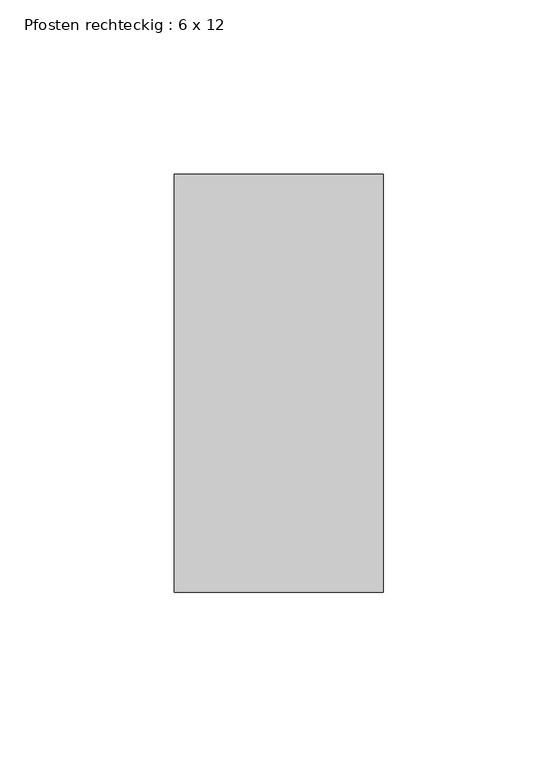
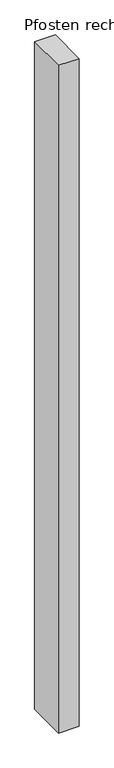
"""IFC4 building model written with IfcOpenShell, lengths in millimetres: member geometry, Pfosten rechteckig : 6 x 12."""

from ifc_helpers import new_model, si_unit, frame, origin, place, context, project, spatial, polyline, outline, extrude, source, transform, mapped, element, save


def pfosten_rechteckig_6_x_12_0a3b7900(model_context):
    return source(origin(), model_context, "Body", "SweptSolid", [
        extrude(outline(polyline([(0.0, 60.0), (0.0, -60.0), (-60.0, -60.0), (-60.0, 60.0), (0.0, 60.0)])), frame((0.0, 0.0, -2050.0000003), z_axis=(0.0, 0.0, 1.0), x_axis=(1.0, 0.0, 0.0)), (0.0, 0.0, 1.0), 2050.0000003),
    ])


if __name__ == "__main__":
    model = new_model("IFC4")
    model_context = context("Model", 3, world=origin())
    ifc_project = project(units=[si_unit("LENGTHUNIT", "METRE", prefix="MILLI")], contexts=[model_context])
    site = spatial("IfcSite", under=ifc_project)
    building = spatial("IfcBuilding", under=site)
    placement = place(None, origin())
    pfosten_rechteckig_6_x_12_shape = pfosten_rechteckig_6_x_12_0a3b7900(model_context)
    element("IfcMember", 1, ObjectType="Pfosten rechteckig : 6 x 12", at=placement, inside=building, context=model_context, shape_type="MappedRepresentation", body=[
        mapped(pfosten_rechteckig_6_x_12_shape, transform((0.0, 0.0, 0.0), x_axis=(1.0, 0.0, 0.0), y_axis=(0.0, 1.0, 0.0), z_axis=(0.0, 0.0, 1.0))),
    ])
    save(model, "model.ifc")

# Revit data of these elements
# Type "Pfosten rechteckig : 6 x 12"
#   built-in parameter 1007304 = 0.393701 (stored number, unit not read)
#   built-in parameter 1007301 = 0.0984252 (stored number, unit not read)
#   built-in parameter 1007300 = 0.0984252 (stored number, unit not read)
# Element 1 (IfcMember, "Pfosten rechteckig : 6 x 12")
#   Materials on its faces: "Metall - verzinkt"
# Materials
#   "Metall - verzinkt": class "Allgemeines", colour RGB 200 200 200, transparency 0, Cost = 0
